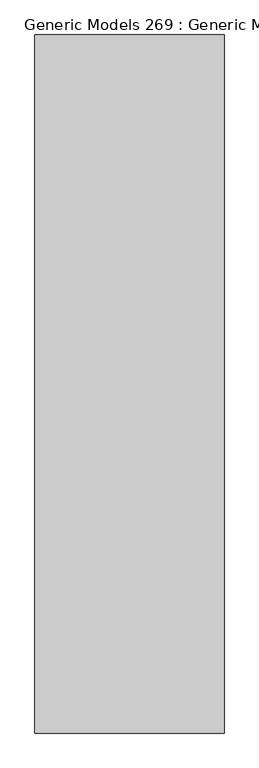
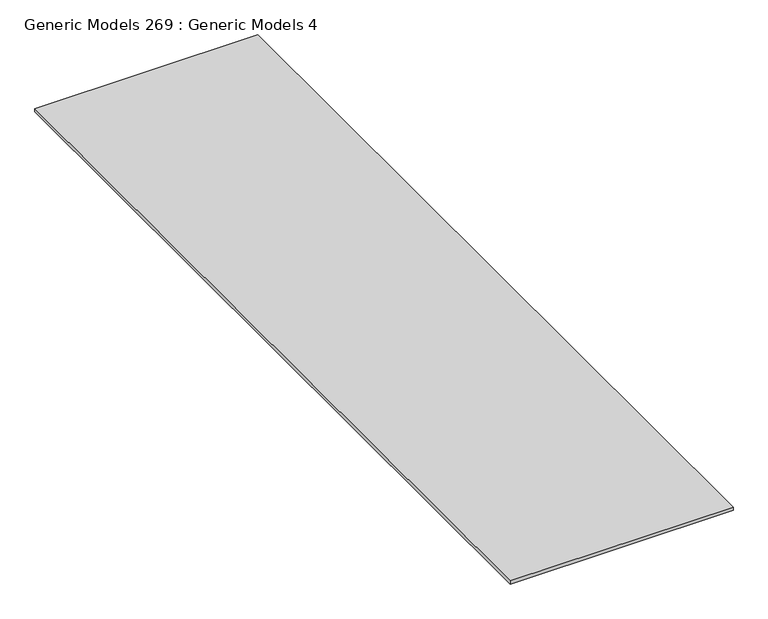
"""IFC4 building model written with IfcOpenShell, lengths in millimetres: proxy geometry, Generic Models 269 : Generic Models 4."""

import ifcopenshell
import ifcopenshell.guid

model = None  # the IFC model being written
_history = None  # IfcOwnerHistory: only IFC2X3 demands one
_inside = {}  # id of a spatial element -> (the spatial element, [elements in it])
_under = {}  # id of a project, library or spatial element -> (it, [spatial elements below it])
_declared = {}  # id of a project -> (the project, [libraries it declares])
_typed = {}  # id of a type object -> (the type object, [elements of that type])
_made_of = {}  # id of a material, layer set ... -> (it, [elements and type objects made of it])


def new_model(schema):
    """Start an empty IFC model of exactly this schema.

    Asked for "IFC4X3", IfcOpenShell would pick the latest addendum, in which some entities
    have other attributes; the version numbers below select the first issue.
    IFC2X3 requires an IfcOwnerHistory on every rooted entity: one is made here for all.
    """
    global model, _history
    if schema == "IFC4X3":
        model = ifcopenshell.file(schema_version=(4, 3, 0, 0))
    else:
        model = ifcopenshell.file(schema=schema)
    _inside.clear()
    _under.clear()
    _declared.clear()
    _typed.clear()
    _made_of.clear()
    _history = None
    if model.schema == "IFC2X3":
        org = make("IfcOrganization", Name="unknown")
        user = make(
            "IfcPersonAndOrganization",
            ThePerson=make("IfcPerson", FamilyName="unknown"),
            TheOrganization=org,
        )
        app = make(
            "IfcApplication",
            ApplicationDeveloper=org,
            Version="unknown",
            ApplicationFullName="unknown",
            ApplicationIdentifier="unknown",
        )
        _history = make(
            "IfcOwnerHistory",
            OwningUser=user,
            OwningApplication=app,
            ChangeAction="ADDED",
            CreationDate=0,
        )
    return model


def make(cls, **values):
    """One entity of the class cls with the attributes given. An attribute that is None is left unset."""
    return model.create_entity(
        cls, **{name: value for name, value in values.items() if value is not None}
    )


def rooted(cls, **values):
    """An entity with a GlobalId (a new one), such as an element, a storey or a relation."""
    return make(cls, GlobalId=ifcopenshell.guid.new(), OwnerHistory=_history, **values)


def si_unit(unit_type, name, prefix=None):
    """IfcSIUnit, for example si_unit("LENGTHUNIT", "METRE", prefix="MILLI")."""
    return make("IfcSIUnit", UnitType=unit_type, Prefix=prefix, Name=name)


def assignment(units):
    """IfcUnitAssignment: the units of a project."""
    return None if units is None else make("IfcUnitAssignment", Units=units)


def point(xyz):
    """IfcCartesianPoint."""
    return None if xyz is None else make("IfcCartesianPoint", Coordinates=xyz)


def direction(xyz):
    """IfcDirection."""
    return None if xyz is None else make("IfcDirection", DirectionRatios=xyz)


def frame(location, z_axis=None, x_axis=None):
    """IfcAxis2Placement3D, a coordinate frame: its origin and axes. An axis left out is left unset."""
    return make(
        "IfcAxis2Placement3D",
        Location=point(location),
        Axis=direction(z_axis),
        RefDirection=direction(x_axis),
    )


def origin():
    """The frame at (0, 0, 0) with its axes left unset."""
    return frame((0.0, 0.0, 0.0))


def place(relative_to, where):
    """IfcLocalPlacement: puts the frame where relative to a parent placement (None: the world)."""
    return make(
        "IfcLocalPlacement", PlacementRelTo=relative_to, RelativePlacement=where
    )


def context(
    kind, dimensions, precision=None, world=None, true_north=None, identifier=None
):
    """IfcGeometricRepresentationContext, for example the 3D "Model" context."""
    return make(
        "IfcGeometricRepresentationContext",
        ContextIdentifier=identifier,
        ContextType=kind,
        CoordinateSpaceDimension=dimensions,
        Precision=precision,
        WorldCoordinateSystem=world,
        TrueNorth=true_north,
    )


def project(units=None, contexts=None):
    """IfcProject with its units and contexts."""
    return rooted(
        "IfcProject",
        Name="project",
        RepresentationContexts=contexts,
        UnitsInContext=assignment(units),
    )


def spatial(cls, under=None, at=None, **own):
    """A site, building, storey or space (cls), placed at a placement, below another one or the project."""
    s = rooted(cls, ObjectPlacement=at, **own)
    if under is not None:
        _under.setdefault(under.id(), (under, []))[1].append(s)
    return s


def polyline(points):
    """IfcPolyline through the points."""
    return make("IfcPolyline", Points=[point(p) for p in points])


def outline(outer, holes=None, kind="AREA"):
    """IfcArbitraryClosedProfileDef: a profile drawn as a closed curve; with holes, ...WithVoids."""
    if holes is None:
        return make("IfcArbitraryClosedProfileDef", ProfileType=kind, OuterCurve=outer)
    return make(
        "IfcArbitraryProfileDefWithVoids",
        ProfileType=kind,
        OuterCurve=outer,
        InnerCurves=holes,
    )


def extrude(swept, where, along, depth):
    """IfcExtrudedAreaSolid: the profile swept, set in the frame where, extruded along a direction by depth."""
    return make(
        "IfcExtrudedAreaSolid",
        SweptArea=swept,
        Position=where,
        ExtrudedDirection=direction(along),
        Depth=depth,
    )


def shape(context_of_items, identifier, shape_type, items):
    """IfcShapeRepresentation: the items that make up one representation, for example the "Body"."""
    return make(
        "IfcShapeRepresentation",
        ContextOfItems=context_of_items,
        RepresentationIdentifier=identifier,
        RepresentationType=shape_type,
        Items=items,
    )


def source(mapping_origin, context_of_items, identifier, shape_type, items):
    """IfcRepresentationMap: a shape defined once, which mapped items show again and again."""
    return make(
        "IfcRepresentationMap",
        MappingOrigin=mapping_origin,
        MappedRepresentation=shape(context_of_items, identifier, shape_type, items),
    )


def transform(
    local_origin,
    x_axis=None,
    y_axis=None,
    z_axis=None,
    scale=None,
    scale2=None,
    scale3=None,
    uniform=True,
):
    """IfcCartesianTransformationOperator3D, or its non-uniform kind. x_axis, y_axis, z_axis: its Axis1, 2, 3."""
    if uniform:
        return make(
            "IfcCartesianTransformationOperator3D",
            Axis1=direction(x_axis),
            Axis2=direction(y_axis),
            LocalOrigin=point(local_origin),
            Scale=scale,
            Axis3=direction(z_axis),
        )
    return make(
        "IfcCartesianTransformationOperator3DnonUniform",
        Axis1=direction(x_axis),
        Axis2=direction(y_axis),
        LocalOrigin=point(local_origin),
        Scale=scale,
        Axis3=direction(z_axis),
        Scale2=scale2,
        Scale3=scale3,
    )


def mapped(mapping_source, mapping_target):
    """IfcMappedItem: shows the shape of a source again, moved by a transform."""
    return make(
        "IfcMappedItem", MappingSource=mapping_source, MappingTarget=mapping_target
    )


def made_of(thing, what):
    """Note that an element or type object is made of a material, layer set ...; save() writes the relation."""
    if what is not None:
        _made_of.setdefault(what.id(), (what, []))[1].append(thing)
    return thing


def element(
    cls,
    number,
    at=None,
    inside=None,
    cuts=None,
    type_object=None,
    material=None,
    context=None,
    identifier="Body",
    shape_type=None,
    held_by="IfcProductDefinitionShape",
    body=None,
    shapes=None,
    **own,
):
    """One element of the class cls, such as IfcWall. Its Tag is "e" and its number.

    at: its placement. inside: the storey or other place that contains it. cuts: it is an
    opening in that element (IfcRelVoidsElement). A single representation is given by context,
    identifier, shape_type and body (its items); several are given by shapes. held_by: the class
    of the entity that holds the representations. save() writes the other relations.
    """
    e = rooted(cls, Tag="e%d" % number, ObjectPlacement=at, **own)
    if body is not None:
        shapes = [shape(context, identifier, shape_type, body)]
    if shapes is not None:
        e.Representation = make(held_by, Representations=shapes)
    if inside is not None:
        _inside.setdefault(inside.id(), (inside, []))[1].append(e)
    if cuts is not None:
        rooted(
            "IfcRelVoidsElement", RelatingBuildingElement=cuts, RelatedOpeningElement=e
        )
    if type_object is not None:
        _typed.setdefault(type_object.id(), (type_object, []))[1].append(e)
    return made_of(e, material)


def aggregate(whole, parts):
    """IfcRelAggregates: a whole, such as a stair, and the parts it consists of."""
    return rooted("IfcRelAggregates", RelatingObject=whole, RelatedObjects=parts)


def save(model, path):
    """Write the relations noted so far, then the file.

    IfcRelAggregates (storeys below a building ...), IfcRelContainedInSpatialStructure (elements
    in a storey), IfcRelDefinesByType, IfcRelAssociatesMaterial and IfcRelDeclares: one each for
    every whole, place, type object, material and project.
    """
    for whole, parts in _under.values():
        aggregate(whole, parts)
    for where, things in _inside.values():
        rooted(
            "IfcRelContainedInSpatialStructure",
            RelatedElements=things,
            RelatingStructure=where,
        )
    for kind, things in _typed.values():
        rooted("IfcRelDefinesByType", RelatedObjects=things, RelatingType=kind)
    for what, things in _made_of.values():
        rooted("IfcRelAssociatesMaterial", RelatedObjects=things, RelatingMaterial=what)
    for by, libraries in _declared.values():
        rooted("IfcRelDeclares", RelatingContext=by, RelatedDefinitions=libraries)
    model.write(path)


def generic_models_269_generic_models_4_02509506(model_context):
    return source(origin(), model_context, "Body", "SweptSolid", [
        extrude(outline(polyline([(-6629.5736296, -5493.3230338), (-10028.1472239, -5493.3230338), (-10028.1472239, 7054.2769662), (-6629.5736296, 7054.2769662), (-6629.5736296, -5493.3230338)])), frame((0.0, 0.0, 122904.8484874), z_axis=(0.0, 0.0, 1.0), x_axis=(1.0, 0.0, 0.0)), (0.0, 0.0, 1.0), 50.8),
    ])


if __name__ == "__main__":
    model = new_model("IFC4")
    model_context = context("Model", 3, world=origin())
    ifc_project = project(units=[si_unit("LENGTHUNIT", "METRE", prefix="MILLI")], contexts=[model_context])
    site = spatial("IfcSite", under=ifc_project)
    building = spatial("IfcBuilding", under=site)
    placement = place(None, origin())
    generic_models_269_generic_models_4_shape = generic_models_269_generic_models_4_02509506(model_context)
    element("IfcBuildingElementProxy", 1, Name="Generic Models 269 : Generic Models 4", ObjectType="Generic Models 269 : Generic Models 4", at=placement, inside=building, context=model_context, shape_type="MappedRepresentation", body=[
        mapped(generic_models_269_generic_models_4_shape, transform((0.0, 0.0, 0.0), x_axis=(1.0, 0.0, 0.0), y_axis=(0.0, 1.0, 0.0), z_axis=(0.0, 0.0, 1.0))),
    ])
    save(model, "model.ifc")

# Revit data of these elements
# Element 1 (IfcBuildingElementProxy, "Generic Models 269 : Generic Models 4")
#   Materials on its faces: "_2\" SAND"
# Materials
#   "_2\" SAND": class "Generic", colour RGB 245 226 173, transparency 0, Cost = 0
